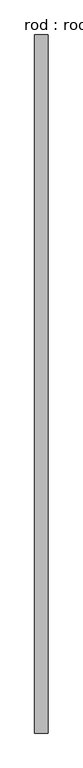
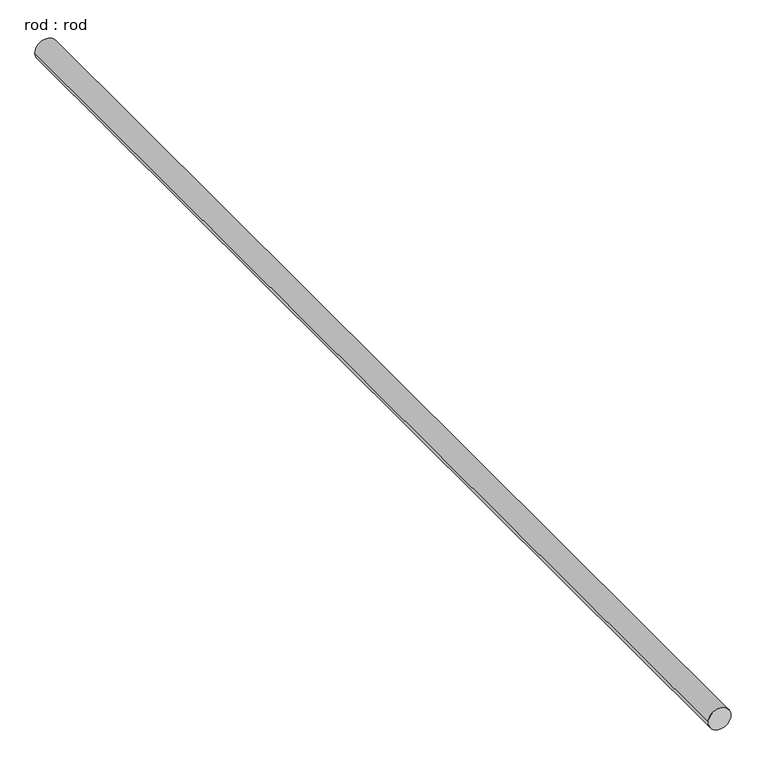
"""IFC4 building model written with IfcOpenShell, lengths in millimetres: proxy geometry, rod : rod."""

from ifc_helpers import new_model, si_unit, point, frame, frame_2d, origin, place, context, project, spatial, circle_curve, trimmed, segment, composite_curve, outline, extrude, source, transform, mapped, element, save


def rod_rod_f27f5d82(model_context):
    return source(origin(), model_context, "Body", "SweptSolid", [
        extrude(outline(composite_curve([segment(trimmed(circle_curve(frame_2d((0.0108462, 0.0)), 200.0), [point((0.0108462, 200.0))], [point((0.0108462, -200.0))], False, "CARTESIAN"), True, "CONTINUOUS"), segment(trimmed(circle_curve(frame_2d((0.0108462, 0.0)), 200.0), [point((0.0108462, -200.0))], [point((0.0108462, 200.0))], False, "CARTESIAN"), True, "CONTINUOUS")], self_intersect=False)), frame((0.0, -6273.3428132, 0.0), z_axis=(0.0, 1.0, 0.0), x_axis=(0.0, 0.0, 1.0)), (0.0, 0.0, 1.0), 20732.1428571),
    ])


if __name__ == "__main__":
    model = new_model("IFC4")
    model_context = context("Model", 3, world=origin())
    ifc_project = project(units=[si_unit("LENGTHUNIT", "METRE", prefix="MILLI")], contexts=[model_context])
    site = spatial("IfcSite", under=ifc_project)
    building = spatial("IfcBuilding", under=site)
    placement = place(None, origin())
    rod_rod_shape = rod_rod_f27f5d82(model_context)
    element("IfcBuildingElementProxy", 1, Name="rod : rod", ObjectType="rod : rod", at=placement, inside=building, context=model_context, shape_type="MappedRepresentation", body=[
        mapped(rod_rod_shape, transform((0.0, 0.0, 0.0), x_axis=(1.0, 0.0, 0.0), y_axis=(0.0, 1.0, 0.0), z_axis=(0.0, 0.0, 1.0))),
    ])
    save(model, "model.ifc")

# Revit data of these elements
# Type "rod : rod"
#   Default Elevation = 0
